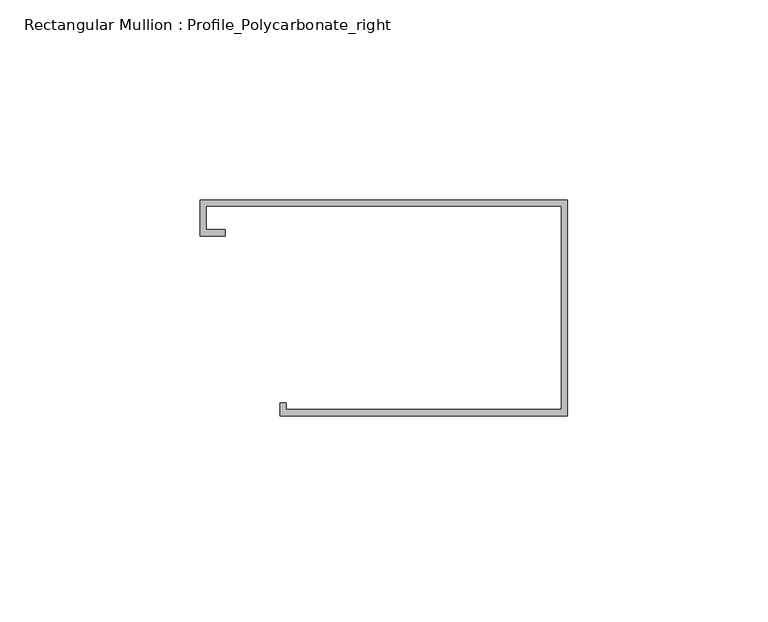
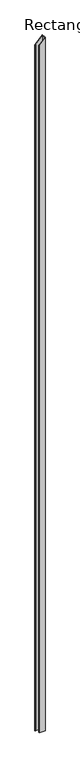
"""IFC4 building model written with IfcOpenShell, lengths in millimetres: member geometry, Rectangular Mullion : Profile_Polycarbonate_right."""

import ifcopenshell
import ifcopenshell.guid

model = None  # the IFC model being written
_history = None  # IfcOwnerHistory: only IFC2X3 demands one
_inside = {}  # id of a spatial element -> (the spatial element, [elements in it])
_under = {}  # id of a project, library or spatial element -> (it, [spatial elements below it])
_declared = {}  # id of a project -> (the project, [libraries it declares])
_typed = {}  # id of a type object -> (the type object, [elements of that type])
_made_of = {}  # id of a material, layer set ... -> (it, [elements and type objects made of it])


def new_model(schema):
    """Start an empty IFC model of exactly this schema.

    Asked for "IFC4X3", IfcOpenShell would pick the latest addendum, in which some entities
    have other attributes; the version numbers below select the first issue.
    IFC2X3 requires an IfcOwnerHistory on every rooted entity: one is made here for all.
    """
    global model, _history
    if schema == "IFC4X3":
        model = ifcopenshell.file(schema_version=(4, 3, 0, 0))
    else:
        model = ifcopenshell.file(schema=schema)
    _inside.clear()
    _under.clear()
    _declared.clear()
    _typed.clear()
    _made_of.clear()
    _history = None
    if model.schema == "IFC2X3":
        org = make("IfcOrganization", Name="unknown")
        user = make(
            "IfcPersonAndOrganization",
            ThePerson=make("IfcPerson", FamilyName="unknown"),
            TheOrganization=org,
        )
        app = make(
            "IfcApplication",
            ApplicationDeveloper=org,
            Version="unknown",
            ApplicationFullName="unknown",
            ApplicationIdentifier="unknown",
        )
        _history = make(
            "IfcOwnerHistory",
            OwningUser=user,
            OwningApplication=app,
            ChangeAction="ADDED",
            CreationDate=0,
        )
    return model


def make(cls, **values):
    """One entity of the class cls with the attributes given. An attribute that is None is left unset."""
    return model.create_entity(
        cls, **{name: value for name, value in values.items() if value is not None}
    )


def rooted(cls, **values):
    """An entity with a GlobalId (a new one), such as an element, a storey or a relation."""
    return make(cls, GlobalId=ifcopenshell.guid.new(), OwnerHistory=_history, **values)


def si_unit(unit_type, name, prefix=None):
    """IfcSIUnit, for example si_unit("LENGTHUNIT", "METRE", prefix="MILLI")."""
    return make("IfcSIUnit", UnitType=unit_type, Prefix=prefix, Name=name)


def assignment(units):
    """IfcUnitAssignment: the units of a project."""
    return None if units is None else make("IfcUnitAssignment", Units=units)


def point(xyz):
    """IfcCartesianPoint."""
    return None if xyz is None else make("IfcCartesianPoint", Coordinates=xyz)


def direction(xyz):
    """IfcDirection."""
    return None if xyz is None else make("IfcDirection", DirectionRatios=xyz)


def frame(location, z_axis=None, x_axis=None):
    """IfcAxis2Placement3D, a coordinate frame: its origin and axes. An axis left out is left unset."""
    return make(
        "IfcAxis2Placement3D",
        Location=point(location),
        Axis=direction(z_axis),
        RefDirection=direction(x_axis),
    )


def origin():
    """The frame at (0, 0, 0) with its axes left unset."""
    return frame((0.0, 0.0, 0.0))


def place(relative_to, where):
    """IfcLocalPlacement: puts the frame where relative to a parent placement (None: the world)."""
    return make(
        "IfcLocalPlacement", PlacementRelTo=relative_to, RelativePlacement=where
    )


def context(
    kind, dimensions, precision=None, world=None, true_north=None, identifier=None
):
    """IfcGeometricRepresentationContext, for example the 3D "Model" context."""
    return make(
        "IfcGeometricRepresentationContext",
        ContextIdentifier=identifier,
        ContextType=kind,
        CoordinateSpaceDimension=dimensions,
        Precision=precision,
        WorldCoordinateSystem=world,
        TrueNorth=true_north,
    )


def project(units=None, contexts=None):
    """IfcProject with its units and contexts."""
    return rooted(
        "IfcProject",
        Name="project",
        RepresentationContexts=contexts,
        UnitsInContext=assignment(units),
    )


def spatial(cls, under=None, at=None, **own):
    """A site, building, storey or space (cls), placed at a placement, below another one or the project."""
    s = rooted(cls, ObjectPlacement=at, **own)
    if under is not None:
        _under.setdefault(under.id(), (under, []))[1].append(s)
    return s


def faces_of(points, faces, orient=None, outer=None):
    """IfcFace entities. A face is a list of loops; a loop is a list of indices into points, from 0.

    orient and outer hold one flag for each loop. By default every Orientation is true, the
    first loop of a face is its IfcFaceOuterBound and the others are IfcFaceBound.
    """
    made = []
    for i, loops in enumerate(faces):
        bounds = []
        for j, loop in enumerate(loops):
            is_outer = j == 0 if outer is None else outer[i][j]
            bounds.append(
                make(
                    "IfcFaceOuterBound" if is_outer else "IfcFaceBound",
                    Bound=make("IfcPolyLoop", Polygon=[points[k] for k in loop]),
                    Orientation=True if orient is None else orient[i][j],
                )
            )
        made.append(make("IfcFace", Bounds=bounds))
    return made


def faceted_brep(points, faces, orient=None, outer=None, voids=None):
    """IfcFacetedBrep: a solid bounded by flat faces; with voids (closed shells), ...WithVoids."""
    shared = [point(p) for p in points]
    hull = make("IfcClosedShell", CfsFaces=faces_of(shared, faces, orient, outer))
    if voids is None:
        return make("IfcFacetedBrep", Outer=hull)
    return make(
        "IfcFacetedBrepWithVoids",
        Outer=hull,
        Voids=[
            make(cls, CfsFaces=faces_of(shared, fs, o, b)) for cls, fs, o, b in voids
        ],
    )


def shape(context_of_items, identifier, shape_type, items):
    """IfcShapeRepresentation: the items that make up one representation, for example the "Body"."""
    return make(
        "IfcShapeRepresentation",
        ContextOfItems=context_of_items,
        RepresentationIdentifier=identifier,
        RepresentationType=shape_type,
        Items=items,
    )


def source(mapping_origin, context_of_items, identifier, shape_type, items):
    """IfcRepresentationMap: a shape defined once, which mapped items show again and again."""
    return make(
        "IfcRepresentationMap",
        MappingOrigin=mapping_origin,
        MappedRepresentation=shape(context_of_items, identifier, shape_type, items),
    )


def transform(
    local_origin,
    x_axis=None,
    y_axis=None,
    z_axis=None,
    scale=None,
    scale2=None,
    scale3=None,
    uniform=True,
):
    """IfcCartesianTransformationOperator3D, or its non-uniform kind. x_axis, y_axis, z_axis: its Axis1, 2, 3."""
    if uniform:
        return make(
            "IfcCartesianTransformationOperator3D",
            Axis1=direction(x_axis),
            Axis2=direction(y_axis),
            LocalOrigin=point(local_origin),
            Scale=scale,
            Axis3=direction(z_axis),
        )
    return make(
        "IfcCartesianTransformationOperator3DnonUniform",
        Axis1=direction(x_axis),
        Axis2=direction(y_axis),
        LocalOrigin=point(local_origin),
        Scale=scale,
        Axis3=direction(z_axis),
        Scale2=scale2,
        Scale3=scale3,
    )


def mapped(mapping_source, mapping_target):
    """IfcMappedItem: shows the shape of a source again, moved by a transform."""
    return make(
        "IfcMappedItem", MappingSource=mapping_source, MappingTarget=mapping_target
    )


def made_of(thing, what):
    """Note that an element or type object is made of a material, layer set ...; save() writes the relation."""
    if what is not None:
        _made_of.setdefault(what.id(), (what, []))[1].append(thing)
    return thing


def element(
    cls,
    number,
    at=None,
    inside=None,
    cuts=None,
    type_object=None,
    material=None,
    context=None,
    identifier="Body",
    shape_type=None,
    held_by="IfcProductDefinitionShape",
    body=None,
    shapes=None,
    **own,
):
    """One element of the class cls, such as IfcWall. Its Tag is "e" and its number.

    at: its placement. inside: the storey or other place that contains it. cuts: it is an
    opening in that element (IfcRelVoidsElement). A single representation is given by context,
    identifier, shape_type and body (its items); several are given by shapes. held_by: the class
    of the entity that holds the representations. save() writes the other relations.
    """
    e = rooted(cls, Tag="e%d" % number, ObjectPlacement=at, **own)
    if body is not None:
        shapes = [shape(context, identifier, shape_type, body)]
    if shapes is not None:
        e.Representation = make(held_by, Representations=shapes)
    if inside is not None:
        _inside.setdefault(inside.id(), (inside, []))[1].append(e)
    if cuts is not None:
        rooted(
            "IfcRelVoidsElement", RelatingBuildingElement=cuts, RelatedOpeningElement=e
        )
    if type_object is not None:
        _typed.setdefault(type_object.id(), (type_object, []))[1].append(e)
    return made_of(e, material)


def aggregate(whole, parts):
    """IfcRelAggregates: a whole, such as a stair, and the parts it consists of."""
    return rooted("IfcRelAggregates", RelatingObject=whole, RelatedObjects=parts)


def save(model, path):
    """Write the relations noted so far, then the file.

    IfcRelAggregates (storeys below a building ...), IfcRelContainedInSpatialStructure (elements
    in a storey), IfcRelDefinesByType, IfcRelAssociatesMaterial and IfcRelDeclares: one each for
    every whole, place, type object, material and project.
    """
    for whole, parts in _under.values():
        aggregate(whole, parts)
    for where, things in _inside.values():
        rooted(
            "IfcRelContainedInSpatialStructure",
            RelatedElements=things,
            RelatingStructure=where,
        )
    for kind, things in _typed.values():
        rooted("IfcRelDefinesByType", RelatedObjects=things, RelatingType=kind)
    for what, things in _made_of.values():
        rooted("IfcRelAssociatesMaterial", RelatedObjects=things, RelatingMaterial=what)
    for by, libraries in _declared.values():
        rooted("IfcRelDeclares", RelatingContext=by, RelatedDefinitions=libraries)
    model.write(path)


def rectangular_mullion_profile_polycarbonate_right_d874f13f(model_context):
    return source(origin(), model_context, "Body", "Brep", [
        faceted_brep([(0.0, 28.984575, -8914.9662617), (0.0, -25.015825, -8914.9662617), (-71.9836, -25.015825, -8914.9662617), (-71.9836, -21.840825, -8914.9662617), (-70.3961, -21.840825, -8914.9662617), (-70.3961, -23.428325, -8914.9662617), (-1.5875, -23.428325, -8914.9662617), (-1.5875, 27.397075, -8914.9662617), (-90.4113, 27.397075, -8914.9662617), (-90.4113, 21.580475, -8914.9662617), (-85.6488, 21.580475, -8914.9662617), (-85.6488, 19.992975, -8914.9662617), (-91.9988, 19.992975, -8914.9662617), (-91.9988, 28.984575, -8914.9662617), (-91.9988, 28.984575, -95.9119088), (0.0, 28.984575, 0.0), (-91.9988, 19.992975, -95.9119088), (-85.6488, 19.992975, -89.2918157), (-85.6488, 21.580475, -89.2918157), (-90.4113, 21.580475, -94.2568855), (-90.4113, 27.397075, -94.2568855), (-1.5875, 27.397075, -1.6550233), (-1.5875, -23.428325, -1.6550233), (-70.3961, -23.428325, -73.3903521), (-70.3961, -21.840825, -73.3903521), (-71.9836, -21.840825, -75.0453753), (-71.9836, -25.015825, -75.0453753), (0.0, -25.015825, 0.0)], [[[0, 1, 2, 3, 4, 5, 6, 7, 8, 9, 10, 11, 12, 13]], [[14, 15, 0, 13]], [[16, 14, 13, 12]], [[17, 16, 12, 11]], [[18, 17, 11, 10]], [[19, 18, 10, 9]], [[20, 19, 9, 8]], [[21, 20, 8, 7]], [[22, 21, 7, 6]], [[23, 22, 6, 5]], [[24, 23, 5, 4]], [[25, 24, 4, 3]], [[26, 25, 3, 2]], [[27, 26, 2, 1]], [[15, 27, 1, 0]], [[15, 14, 16, 17, 18, 19, 20, 21, 22, 23, 24, 25, 26, 27]]]),
    ])


if __name__ == "__main__":
    model = new_model("IFC4")
    model_context = context("Model", 3, world=origin())
    ifc_project = project(units=[si_unit("LENGTHUNIT", "METRE", prefix="MILLI")], contexts=[model_context])
    site = spatial("IfcSite", under=ifc_project)
    building = spatial("IfcBuilding", under=site)
    placement = place(None, origin())
    rectangular_mullion_profile_polycarbonate_right_shape = rectangular_mullion_profile_polycarbonate_right_d874f13f(model_context)
    element("IfcMember", 1, ObjectType="Rectangular Mullion : Profile_Polycarbonate_right", at=placement, inside=building, context=model_context, shape_type="MappedRepresentation", body=[
        mapped(rectangular_mullion_profile_polycarbonate_right_shape, transform((0.0, 0.0, 0.0), x_axis=(1.0, 0.0, 0.0), y_axis=(0.0, 1.0, 0.0), z_axis=(0.0, 0.0, 1.0))),
    ])
    save(model, "model.ifc")

# Revit data of these elements
# Type "Rectangular Mullion : Profile_Polycarbonate_right"
#   built-in parameter 1007322 = 0.177167 (stored number, unit not read)
#   built-in parameter 1007321 = 0 (stored number, unit not read)
#   built-in parameter 1007320 = 0.00520833 (stored number, unit not read)
